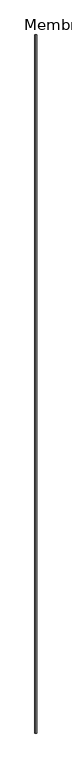
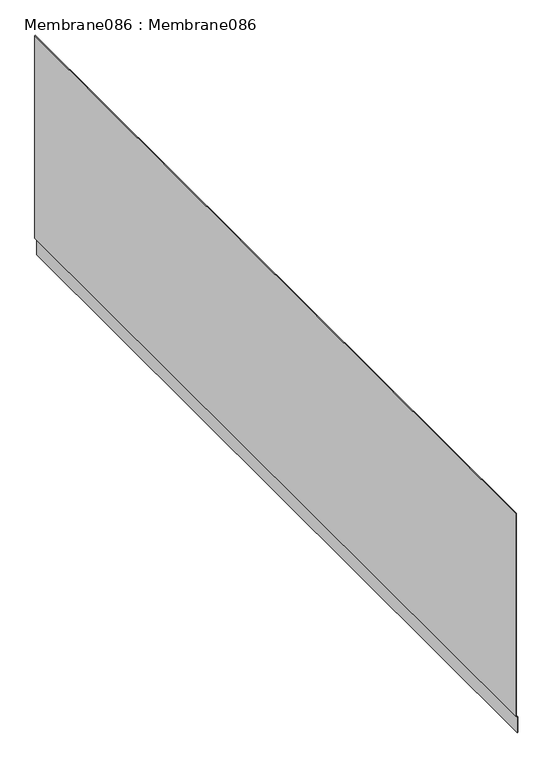
"""IFC4 building model written with IfcOpenShell, lengths in millimetres: proxy geometry, Membrane086 : Membrane086."""

from ifc_helpers import new_model, si_unit, frame, origin, place, context, project, spatial, polyline, outline, extrude, source, transform, mapped, element, save


def membrane086_membrane086_8d3ee5e9(model_context):
    return source(origin(), model_context, "Body", "SweptSolid", [
        extrude(outline(polyline([(40204.1521458, 16506.4283752), (40165.4646458, 16506.4283752), (40165.4646458, 16507.8283752), (40204.7545147, 16507.8283752), (40208.4498272, 16503.9260315), (40722.29602, 16503.9260315), (40722.29602, 16502.5260315), (40207.8474583, 16502.5260315), (40204.1521458, 16506.4283752)])), frame((0.0, -1052.8906567, 0.0), z_axis=(0.0, 1.0, 0.0), x_axis=(0.0, 0.0, 1.0)), (0.0, 0.0, 1.0), 1999.85),
    ])


if __name__ == "__main__":
    model = new_model("IFC4")
    model_context = context("Model", 3, world=origin())
    ifc_project = project(units=[si_unit("LENGTHUNIT", "METRE", prefix="MILLI")], contexts=[model_context])
    site = spatial("IfcSite", under=ifc_project)
    building = spatial("IfcBuilding", under=site)
    placement = place(None, origin())
    membrane086_membrane086_shape = membrane086_membrane086_8d3ee5e9(model_context)
    element("IfcBuildingElementProxy", 1, Name="Membrane086 : Membrane086", ObjectType="Membrane086 : Membrane086", at=placement, inside=building, context=model_context, shape_type="MappedRepresentation", body=[
        mapped(membrane086_membrane086_shape, transform((0.0, 0.0, 0.0), x_axis=(1.0, 0.0, 0.0), y_axis=(0.0, 1.0, 0.0), z_axis=(0.0, 0.0, 1.0))),
    ])
    save(model, "model.ifc")

# Revit data of these elements
# Type "Membrane086 : Membrane086"
#   NameOverride = "Membrane086"
# Element 1 (IfcBuildingElementProxy, "Membrane086 : Membrane086")
#   Materials on its faces: "(2) LAYERS OF ICE & WATER SHIELD (BITUTHANE) UNDER STUCCO"
# Materials
#   "(2) LAYERS OF ICE & WATER SHIELD (BITUTHANE) UNDER STUCCO": class "Unassigned", colour RGB 186 255 159, transparency 0, Cost = 0
